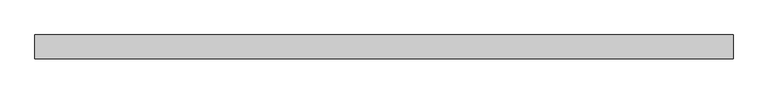
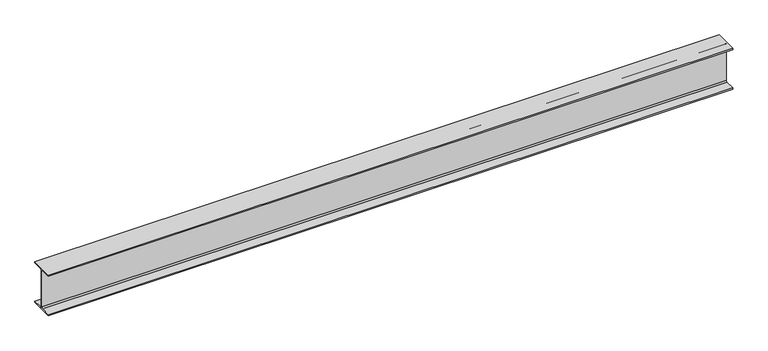
"""IFC4 building model written with IfcOpenShell, lengths in millimetres: beam geometry, Old_Steel Beam_H-KSD3502 : H_SB_ASB_H-250×125x6x9."""

from ifc_helpers import new_model, si_unit, point, frame, frame_2d, origin, place, context, project, spatial, polyline, circle_curve, trimmed, segment, composite_curve, outline, extrude, source, transform, mapped, element, save


def beam_19858f58(model_context):
    return source(origin(), model_context, "Body", "SweptSolid", [
        extrude(outline(composite_curve([segment(polyline([(82.5, -141.5), (82.5, -151.7), (-82.5, -151.7), (-82.5, -141.5), (-11.9, -141.5)]), True, "CONTINUOUS"), segment(trimmed(circle_curve(frame_2d((-11.9, -132.6)), 8.9), [point((-11.9, -141.5))], [point((-3.0, -132.6))], True, "CARTESIAN"), True, "CONTINUOUS"), segment(polyline([(-3.0, -132.6), (-3.0, 132.6)]), True, "CONTINUOUS"), segment(trimmed(circle_curve(frame_2d((-11.9, 132.6)), 8.9), [point((-3.0, 132.6))], [point((-11.9, 141.5))], True, "CARTESIAN"), True, "CONTINUOUS"), segment(polyline([(-11.9, 141.5), (-82.5, 141.5), (-82.5, 151.7), (82.5, 151.7), (82.5, 141.5), (11.9, 141.5)]), True, "CONTINUOUS"), segment(trimmed(circle_curve(frame_2d((11.9, 132.6)), 8.9), [point((11.9, 141.5))], [point((3.0, 132.6))], True, "CARTESIAN"), True, "CONTINUOUS"), segment(polyline([(3.0, 132.6), (3.0, -132.6)]), True, "CONTINUOUS"), segment(trimmed(circle_curve(frame_2d((11.9, -132.6)), 8.9), [point((3.0, -132.6))], [point((11.9, -141.5))], True, "CARTESIAN"), True, "CONTINUOUS"), segment(polyline([(11.9, -141.5), (82.5, -141.5)]), True, "CONTINUOUS")], self_intersect=False)), frame((-2404.8281705, 0.0, 0.0), z_axis=(1.0, 0.0, 0.0), x_axis=(0.0, 1.0, 0.0)), (0.0, 0.0, 1.0), 4808.1916513),
    ])


if __name__ == "__main__":
    model = new_model("IFC4")
    model_context = context("Model", 3, world=origin())
    ifc_project = project(units=[si_unit("LENGTHUNIT", "METRE", prefix="MILLI")], contexts=[model_context])
    site = spatial("IfcSite", under=ifc_project)
    building = spatial("IfcBuilding", under=site)
    placement = place(None, origin())
    beam_shape = beam_19858f58(model_context)
    element("IfcBeam", 1, ObjectType="Old_Steel Beam_H-KSD3502 : H_SB_ASB_H-250×125x6x9", at=placement, inside=building, context=model_context, shape_type="MappedRepresentation", body=[
        mapped(beam_shape, transform((0.0, 0.0, 0.0), x_axis=(1.0, 0.0, 0.0), y_axis=(0.0, 1.0, 0.0), z_axis=(0.0, 0.0, 1.0))),
    ])
    save(model, "model.ifc")

# Revit data of these elements
# Type "Old_Steel Beam_H-KSD3502 : H_SB_ASB_H-250×125x6x9"
#   Width = 12.5 cm
#   Web Thickness = 0.6 cm
#   Web Fillet = 1.2 cm
#   Warping Constant = 42539.8 cm⁶
#   Torsional Moment of Inertia = 7.8102 cm⁴
#   Torsional Modulus = 1.0 cm³
#   Section Area = 37.66 cm²
#   Plastic Modulus weak axis = 73.1 cm³
#   Plastic Modulus strong axis = 366.0 cm³
#   Perimeter = 0.97 m²/m
#   Nominal Weight = 29.60 kgf/m
#   Moment of Inertia weak axis = 294.00 cm⁴
#   Moment of Inertia strong axis = 4050.00 cm⁴
#   Height = 25.0 cm
#   Flange Thickness = 0.9 cm
#   Elastic Modulus weak axis = 47.0 cm³
#   Elastic Modulus strong axis = 324.0 cm³
#   Centroid Vertical = 12.5 cm
#   Centroid Horizontal = 6.25 cm
#   Length [instance default] = 1.5240 m
#   Structural Material [instance default] = Steel, 45-345
#   Assembly Code = ""
# Element 1 (IfcBeam, "Old_Steel Beam_H-KSD3502 : H_SB_ASB_H-250×125x6x9")
#   Structural Material = none
# Materials
#   "Steel, 45-345": class "Metal", colour RGB 189 187 185, transparency 0, Description = "Steel 345 MPa", Cost = 0
